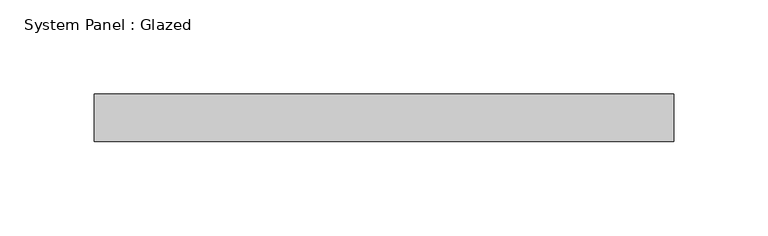
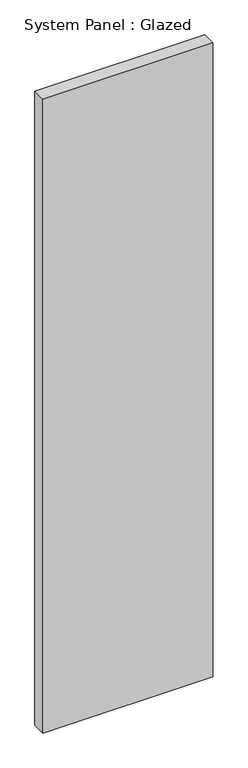
"""IFC4 building model written with IfcOpenShell, lengths in millimetres: plate geometry, System Panel : Glazed."""

from ifc_helpers import new_model, si_unit, origin, origin_with_axes, place, context, project, spatial, polyline, outline, extrude, source, transform, mapped, element, save


def system_panel_glazed_e20ab226(model_context):
    return source(origin(), model_context, "Body", "SweptSolid", [
        extrude(outline(polyline([(153.9999998, 19.05), (-153.9999998, 19.05), (-153.9999998, 44.45), (153.9999998, 44.45), (153.9999998, 19.05)])), origin_with_axes(), (0.0, 0.0, 1.0), 1216.0),
    ])


if __name__ == "__main__":
    model = new_model("IFC4")
    model_context = context("Model", 3, world=origin())
    ifc_project = project(units=[si_unit("LENGTHUNIT", "METRE", prefix="MILLI")], contexts=[model_context])
    site = spatial("IfcSite", under=ifc_project)
    building = spatial("IfcBuilding", under=site)
    placement = place(None, origin())
    system_panel_glazed_shape = system_panel_glazed_e20ab226(model_context)
    element("IfcPlate", 1, ObjectType="System Panel : Glazed", at=placement, inside=building, context=model_context, shape_type="MappedRepresentation", body=[
        mapped(system_panel_glazed_shape, transform((0.0, 0.0, 0.0), x_axis=(1.0, 0.0, 0.0), y_axis=(0.0, 1.0, 0.0), z_axis=(0.0, 0.0, 1.0))),
    ])
    save(model, "model.ifc")

# Revit data of these elements
# Type "System Panel : Glazed"
#   Construction Type Id = "GSP4R"
#   Analytic Construction = "1/8 in Pilkington single glazing"
#   Visual Light Transmittance = 0.9
#   Solar Heat Gain Coefficient = 0.86
#   Heat Transfer Coefficient (U) = 6.7069 W/(m²·K)
# Element 1 (IfcPlate, "System Panel : Glazed")
#   Materials on its faces: "Glass"
# Materials
#   "Glass": class "Glass", colour RGB 0 128 192, transparency 0.75, Description = "Soda Lime Glass", Cost = 0
